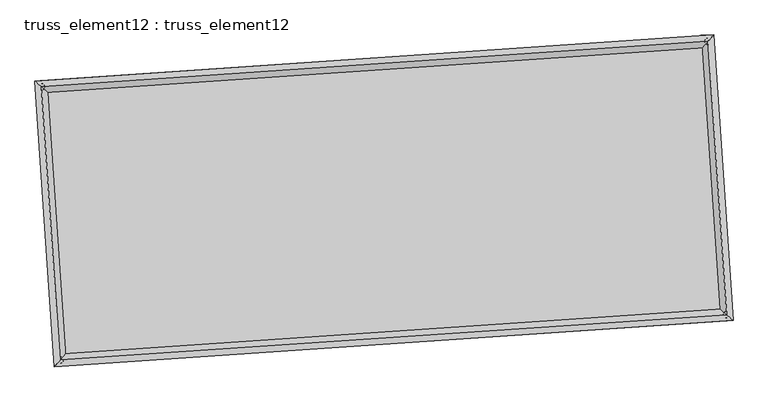
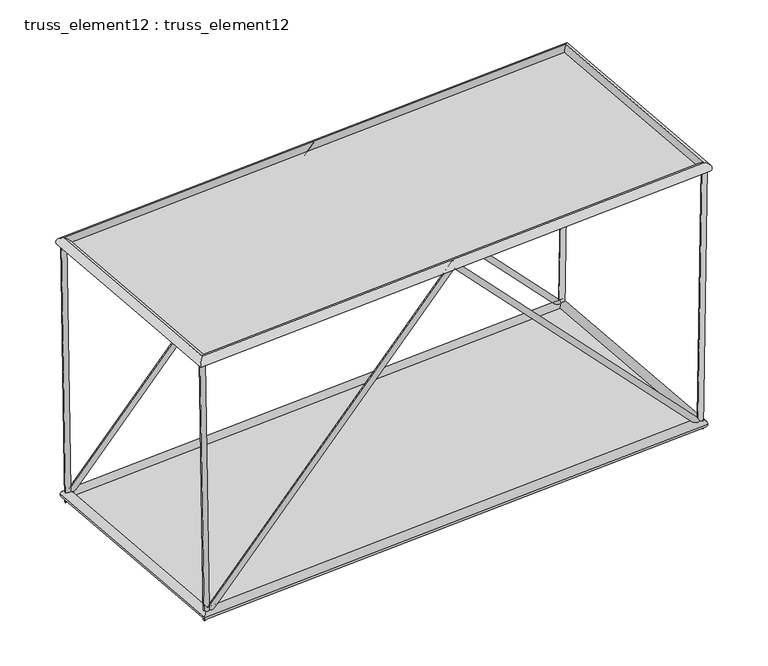
"""IFC4 building model written with IfcOpenShell, lengths in millimetres: plate geometry, truss_element12 : truss_element12."""

import ifcopenshell
import ifcopenshell.guid

model = None  # the IFC model being written
_history = None  # IfcOwnerHistory: only IFC2X3 demands one
_inside = {}  # id of a spatial element -> (the spatial element, [elements in it])
_under = {}  # id of a project, library or spatial element -> (it, [spatial elements below it])
_declared = {}  # id of a project -> (the project, [libraries it declares])
_typed = {}  # id of a type object -> (the type object, [elements of that type])
_made_of = {}  # id of a material, layer set ... -> (it, [elements and type objects made of it])


def new_model(schema):
    """Start an empty IFC model of exactly this schema.

    Asked for "IFC4X3", IfcOpenShell would pick the latest addendum, in which some entities
    have other attributes; the version numbers below select the first issue.
    IFC2X3 requires an IfcOwnerHistory on every rooted entity: one is made here for all.
    """
    global model, _history
    if schema == "IFC4X3":
        model = ifcopenshell.file(schema_version=(4, 3, 0, 0))
    else:
        model = ifcopenshell.file(schema=schema)
    _inside.clear()
    _under.clear()
    _declared.clear()
    _typed.clear()
    _made_of.clear()
    _history = None
    if model.schema == "IFC2X3":
        org = make("IfcOrganization", Name="unknown")
        user = make(
            "IfcPersonAndOrganization",
            ThePerson=make("IfcPerson", FamilyName="unknown"),
            TheOrganization=org,
        )
        app = make(
            "IfcApplication",
            ApplicationDeveloper=org,
            Version="unknown",
            ApplicationFullName="unknown",
            ApplicationIdentifier="unknown",
        )
        _history = make(
            "IfcOwnerHistory",
            OwningUser=user,
            OwningApplication=app,
            ChangeAction="ADDED",
            CreationDate=0,
        )
    return model


def make(cls, **values):
    """One entity of the class cls with the attributes given. An attribute that is None is left unset."""
    return model.create_entity(
        cls, **{name: value for name, value in values.items() if value is not None}
    )


def rooted(cls, **values):
    """An entity with a GlobalId (a new one), such as an element, a storey or a relation."""
    return make(cls, GlobalId=ifcopenshell.guid.new(), OwnerHistory=_history, **values)


def si_unit(unit_type, name, prefix=None):
    """IfcSIUnit, for example si_unit("LENGTHUNIT", "METRE", prefix="MILLI")."""
    return make("IfcSIUnit", UnitType=unit_type, Prefix=prefix, Name=name)


def assignment(units):
    """IfcUnitAssignment: the units of a project."""
    return None if units is None else make("IfcUnitAssignment", Units=units)


def point(xyz):
    """IfcCartesianPoint."""
    return None if xyz is None else make("IfcCartesianPoint", Coordinates=xyz)


def direction(xyz):
    """IfcDirection."""
    return None if xyz is None else make("IfcDirection", DirectionRatios=xyz)


def frame(location, z_axis=None, x_axis=None):
    """IfcAxis2Placement3D, a coordinate frame: its origin and axes. An axis left out is left unset."""
    return make(
        "IfcAxis2Placement3D",
        Location=point(location),
        Axis=direction(z_axis),
        RefDirection=direction(x_axis),
    )


def origin():
    """The frame at (0, 0, 0) with its axes left unset."""
    return frame((0.0, 0.0, 0.0))


def origin_with_axes():
    """The frame at (0, 0, 0) with the z axis (0, 0, 1) and the x axis (1, 0, 0) written out."""
    return frame((0.0, 0.0, 0.0), z_axis=(0.0, 0.0, 1.0), x_axis=(1.0, 0.0, 0.0))


def place(relative_to, where):
    """IfcLocalPlacement: puts the frame where relative to a parent placement (None: the world)."""
    return make(
        "IfcLocalPlacement", PlacementRelTo=relative_to, RelativePlacement=where
    )


def context(
    kind, dimensions, precision=None, world=None, true_north=None, identifier=None
):
    """IfcGeometricRepresentationContext, for example the 3D "Model" context."""
    return make(
        "IfcGeometricRepresentationContext",
        ContextIdentifier=identifier,
        ContextType=kind,
        CoordinateSpaceDimension=dimensions,
        Precision=precision,
        WorldCoordinateSystem=world,
        TrueNorth=true_north,
    )


def project(units=None, contexts=None):
    """IfcProject with its units and contexts."""
    return rooted(
        "IfcProject",
        Name="project",
        RepresentationContexts=contexts,
        UnitsInContext=assignment(units),
    )


def spatial(cls, under=None, at=None, **own):
    """A site, building, storey or space (cls), placed at a placement, below another one or the project."""
    s = rooted(cls, ObjectPlacement=at, **own)
    if under is not None:
        _under.setdefault(under.id(), (under, []))[1].append(s)
    return s


def polyline(points):
    """IfcPolyline through the points."""
    return make("IfcPolyline", Points=[point(p) for p in points])


def circle_curve(where, radius):
    """IfcCircle in the frame where."""
    return make("IfcCircle", Position=where, Radius=radius)


def ellipse_curve(where, semi_axis1, semi_axis2):
    """IfcEllipse in the frame where."""
    return make(
        "IfcEllipse", Position=where, SemiAxis1=semi_axis1, SemiAxis2=semi_axis2
    )


def outline(outer, holes=None, kind="AREA"):
    """IfcArbitraryClosedProfileDef: a profile drawn as a closed curve; with holes, ...WithVoids."""
    if holes is None:
        return make("IfcArbitraryClosedProfileDef", ProfileType=kind, OuterCurve=outer)
    return make(
        "IfcArbitraryProfileDefWithVoids",
        ProfileType=kind,
        OuterCurve=outer,
        InnerCurves=holes,
    )


def extrude(swept, where, along, depth):
    """IfcExtrudedAreaSolid: the profile swept, set in the frame where, extruded along a direction by depth."""
    return make(
        "IfcExtrudedAreaSolid",
        SweptArea=swept,
        Position=where,
        ExtrudedDirection=direction(along),
        Depth=depth,
    )


def shape(context_of_items, identifier, shape_type, items):
    """IfcShapeRepresentation: the items that make up one representation, for example the "Body"."""
    return make(
        "IfcShapeRepresentation",
        ContextOfItems=context_of_items,
        RepresentationIdentifier=identifier,
        RepresentationType=shape_type,
        Items=items,
    )


def source(mapping_origin, context_of_items, identifier, shape_type, items):
    """IfcRepresentationMap: a shape defined once, which mapped items show again and again."""
    return make(
        "IfcRepresentationMap",
        MappingOrigin=mapping_origin,
        MappedRepresentation=shape(context_of_items, identifier, shape_type, items),
    )


def transform(
    local_origin,
    x_axis=None,
    y_axis=None,
    z_axis=None,
    scale=None,
    scale2=None,
    scale3=None,
    uniform=True,
):
    """IfcCartesianTransformationOperator3D, or its non-uniform kind. x_axis, y_axis, z_axis: its Axis1, 2, 3."""
    if uniform:
        return make(
            "IfcCartesianTransformationOperator3D",
            Axis1=direction(x_axis),
            Axis2=direction(y_axis),
            LocalOrigin=point(local_origin),
            Scale=scale,
            Axis3=direction(z_axis),
        )
    return make(
        "IfcCartesianTransformationOperator3DnonUniform",
        Axis1=direction(x_axis),
        Axis2=direction(y_axis),
        LocalOrigin=point(local_origin),
        Scale=scale,
        Axis3=direction(z_axis),
        Scale2=scale2,
        Scale3=scale3,
    )


def mapped(mapping_source, mapping_target):
    """IfcMappedItem: shows the shape of a source again, moved by a transform."""
    return make(
        "IfcMappedItem", MappingSource=mapping_source, MappingTarget=mapping_target
    )


def made_of(thing, what):
    """Note that an element or type object is made of a material, layer set ...; save() writes the relation."""
    if what is not None:
        _made_of.setdefault(what.id(), (what, []))[1].append(thing)
    return thing


def element(
    cls,
    number,
    at=None,
    inside=None,
    cuts=None,
    type_object=None,
    material=None,
    context=None,
    identifier="Body",
    shape_type=None,
    held_by="IfcProductDefinitionShape",
    body=None,
    shapes=None,
    **own,
):
    """One element of the class cls, such as IfcWall. Its Tag is "e" and its number.

    at: its placement. inside: the storey or other place that contains it. cuts: it is an
    opening in that element (IfcRelVoidsElement). A single representation is given by context,
    identifier, shape_type and body (its items); several are given by shapes. held_by: the class
    of the entity that holds the representations. save() writes the other relations.
    """
    e = rooted(cls, Tag="e%d" % number, ObjectPlacement=at, **own)
    if body is not None:
        shapes = [shape(context, identifier, shape_type, body)]
    if shapes is not None:
        e.Representation = make(held_by, Representations=shapes)
    if inside is not None:
        _inside.setdefault(inside.id(), (inside, []))[1].append(e)
    if cuts is not None:
        rooted(
            "IfcRelVoidsElement", RelatingBuildingElement=cuts, RelatedOpeningElement=e
        )
    if type_object is not None:
        _typed.setdefault(type_object.id(), (type_object, []))[1].append(e)
    return made_of(e, material)


def aggregate(whole, parts):
    """IfcRelAggregates: a whole, such as a stair, and the parts it consists of."""
    return rooted("IfcRelAggregates", RelatingObject=whole, RelatedObjects=parts)


def save(model, path):
    """Write the relations noted so far, then the file.

    IfcRelAggregates (storeys below a building ...), IfcRelContainedInSpatialStructure (elements
    in a storey), IfcRelDefinesByType, IfcRelAssociatesMaterial and IfcRelDeclares: one each for
    every whole, place, type object, material and project.
    """
    for whole, parts in _under.values():
        aggregate(whole, parts)
    for where, things in _inside.values():
        rooted(
            "IfcRelContainedInSpatialStructure",
            RelatedElements=things,
            RelatingStructure=where,
        )
    for kind, things in _typed.values():
        rooted("IfcRelDefinesByType", RelatedObjects=things, RelatingType=kind)
    for what, things in _made_of.values():
        rooted("IfcRelAssociatesMaterial", RelatedObjects=things, RelatingMaterial=what)
    for by, libraries in _declared.values():
        rooted("IfcRelDeclares", RelatingContext=by, RelatedDefinitions=libraries)
    model.write(path)


def plane_surface(at):
    """IfcPlane: the flat surface through the origin of the frame at, square to its z axis."""
    return make("IfcPlane", Position=at)


def cylinder_surface(at, radius):
    """IfcCylindricalSurface: all points at the distance radius from the z axis of the frame at."""
    return make("IfcCylindricalSurface", Position=at, Radius=radius)


def advanced_brep(points, edges, surfaces, faces):
    """IfcAdvancedBrep: a solid bounded by faces that lie on surfaces and meet in shared edges.

    An edge is (start, end): straight between two places in points (the first is 0);
    or (start, end, curve); or (start, end, curve, False) where it runs against its curve.
    A face is (place in surfaces, loops), or (place, loops, False) where it looks against
    its surface's normal. A loop lists edges by number (the first is 1), with a minus sign
    where the edge is run from its end to its start. The first loop is the outer one.
    """
    corners = [point(p) for p in points]
    vertices = [make("IfcVertexPoint", VertexGeometry=c) for c in corners]
    made = []
    for start, end, *more in edges:
        made.append(
            make(
                "IfcEdgeCurve",
                EdgeStart=vertices[start],
                EdgeEnd=vertices[end],
                EdgeGeometry=more[0] if more else make("IfcPolyline", Points=[corners[start], corners[end]]),
                SameSense=more[1] if len(more) > 1 else True,
            )
        )
    hull = []
    for where, loops, *sense in faces:
        bounds = []
        for j, loop in enumerate(loops):
            ring = [make("IfcOrientedEdge", EdgeElement=made[abs(k) - 1], Orientation=k > 0) for k in loop]
            bounds.append(
                make(
                    "IfcFaceOuterBound" if j == 0 else "IfcFaceBound",
                    Bound=make("IfcEdgeLoop", EdgeList=ring),
                    Orientation=True,
                )
            )
        hull.append(make("IfcAdvancedFace", Bounds=bounds, FaceSurface=surfaces[where], SameSense=sense[0] if sense else True))
    return make("IfcAdvancedBrep", Outer=make("IfcClosedShell", CfsFaces=hull))


def truss_element12_truss_element12_1bbcfac7(model_context):
    return source(origin(), model_context, "Body", "SolidModel", [
        advanced_brep(
        [(-3746.2779315, 2270.677949, 5000.1488437), (-3845.3680681, 2257.3176242, 4998.522018), (-3666.9216571, 2276.0889517, 122.1113591), (-3762.0652257, 2262.9977284, -122.1113591), (1064.4228838, 2598.7013505, 5071.4427935), (1064.8605805, 2592.1274502, 4927.2050495), (5794.3942317, 2921.2201164, 122.1016693), (5890.3667453, 2921.1603721, -122.1016693), (5875.1134246, 2926.7240513, 5000.1397912), (5975.0995037, 2926.9379768, 4998.4850331)],
        [
            (0, 1, circle_curve(frame((-3795.8229998, 2263.9977866, 4999.3354308), z_axis=(-0.016265911675968303, -0.0011091106846651264, 0.9998670861623754), x_axis=(-0.1336035338535352, 0.9910342788842121, -0.0010741593443196402)), 50.0)),
            (1, 0, circle_curve(frame((-3795.8229998, 2263.9977866, 4999.3354308), z_axis=(-0.016265911675968303, -0.0011091106846651264, 0.9998670861623754), x_axis=(-0.1336035338535352, 0.9910342788842121, -0.0010741593443196402)), 50.0)),
            (0, 2),
            (2, 3, ellipse_curve(frame((-3714.4934414, 2269.54334, 0.0), z_axis=(-0.9287646394568875, -0.06332893019963927, 0.36522005845009003), x_axis=(0.36437398822915085, 0.02484527714214224, 0.9309212151979955)), 131.4582279, 50.0)),
            (3, 1),
            (3, 2, ellipse_curve(frame((-3714.4934414, 2269.54334, 0.0), z_axis=(-0.9287646394568875, -0.06332893019963927, 0.36522005845009003), x_axis=(0.36437398822915085, 0.02484527714214224, 0.9309212151979955)), 131.4582279, 50.0)),
            (2, 4),
            (4, 5, ellipse_curve(frame((1064.6417322, 2595.4144003, 4999.3239215), z_axis=(-0.9976833934171915, -0.06802823804748175, 7.299118212849759e-05), x_axis=(-7.282209046969254e-05, -4.9654615264680074e-06, -0.9999999973361436)), 72.2759091, 50.0)),
            (5, 3),
            (5, 4, ellipse_curve(frame((1064.6417322, 2595.4144003, 4999.3239215), z_axis=(-0.9976833934171915, -0.06802823804748175, 7.299118212849759e-05), x_axis=(-7.282209046969254e-05, -4.9654615264680074e-06, -0.9999999973361436)), 72.2759091, 50.0)),
            (4, 6),
            (6, 7, ellipse_curve(frame((5842.3804885, 2921.1902443, 0.0), z_axis=(-0.9288422213363277, -0.06333422021308223, -0.3650217862169288), x_axis=(-0.3641761753142233, -0.02483178903143046, 0.930998977221244)), 131.4368172, 50.0)),
            (7, 5),
            (7, 6, ellipse_curve(frame((5842.3804885, 2921.1902443, 0.0), z_axis=(-0.9288422213363277, -0.06333422021308223, -0.3650217862169288), x_axis=(-0.3641761753142233, -0.02483178903143046, 0.930998977221244)), 131.4368172, 50.0)),
            (8, 9, circle_curve(frame((5925.1064641, 2926.8310141, 4999.3124122), z_axis=(0.016545195126702994, 0.0011281539615151874, 0.9998624824378893), x_axis=(-0.0021576295961431924, 0.9999970754228623, -0.0010926025114963022)), 50.0)),
            (9, 8, circle_curve(frame((5925.1064641, 2926.8310141, 4999.3124122), z_axis=(0.016545195126702994, 0.0011281539615151874, 0.9998624824378893), x_axis=(-0.0021576295961431924, 0.9999970754228623, -0.0010926025114963022)), 50.0)),
            (6, 8),
            (9, 7),
        ],
        [
            plane_surface(frame((-3795.8229998, 2313.9977559, 4999.3908937), z_axis=(-0.016265911675968123, -0.0011091106846617949, 0.9998670861623753), x_axis=(0.9998677013072027, -1.8043083511720685e-05, 0.01626590166875275))),
            cylinder_surface(frame((-3795.8229998, 2263.9977866, 4999.3354308), z_axis=(-0.016265911675968303, -0.0011091106846651264, 0.9998670861623754), x_axis=(-0.1336035338535352, 0.9910342788842121, -0.0010741593443196402)), 50.0),
            cylinder_surface(frame((-3714.4934414, 2269.54334, 0.0), z_axis=(-0.6902434140818179, -0.04706507454537663, -0.7220449487910807), x_axis=(-0.020419087296308105, 0.9987518960405878, -0.045581915595078945)), 50.0),
            cylinder_surface(frame((1064.6417322, 2595.4144003, 4999.3239215), z_axis=(-0.6901382450820931, -0.04705790347107014, 0.7221459384334419), x_axis=(-0.11534841177711228, 0.9922790262643878, -0.045574970502419106)), 50.0),
            plane_surface(frame((5925.1064641, 2876.8310459, 4999.3688276), z_axis=(0.01654519512670156, 0.0011281539615101215, 0.9998624824378892), x_axis=(0.9998631188908906, -1.8668082734762968e-05, -0.016545184595020874))),
            cylinder_surface(frame((5842.3804885, 2921.1902443, 0.0), z_axis=(-0.016545195126702994, -0.0011281539615151874, -0.9998624824378893), x_axis=(-0.0021576295961431924, 0.9999970754228623, -0.0010926025114963022)), 50.0),
        ],
        [
            (0, [[1, 2]]),
            (1, [[-1, 3, 4, 5]]),
            (1, [[-2, -5, 6, -3]]),
            (2, [[-4, 7, 8, 9]]),
            (2, [[-6, -9, 10, -7]]),
            (3, [[-8, 11, 12, 13]]),
            (3, [[-10, -13, 14, -11]]),
            (4, [[15, 16]]),
            (5, [[-12, 17, -16, 18]]),
            (5, [[-14, -18, -15, -17]]),
        ],
    ),
        advanced_brep(
        [(-3474.1649786, -1720.0556353, 5000.1488437), (-3573.2551151, -1733.4159601, 4998.522018), (-3394.8087042, -1714.6446326, 122.1113591), (-3489.9522728, -1727.7358559, -122.1113591), (1336.5358367, -1392.0322338, 5071.4427935), (1336.9735335, -1398.6061341, 4927.2050495), (6066.5071846, -1069.5134679, 122.1016693), (6162.4796982, -1069.5732122, -122.1016693), (6147.2263775, -1064.009533, 5000.1397912), (6247.2124566, -1063.7956075, 4998.4850331)],
        [
            (0, 1, circle_curve(frame((-3523.7100469, -1726.7357977, 4999.3354308), z_axis=(-0.01626591167596829, -0.0011091106846651422, 0.9998670861623754), x_axis=(-0.13360353385353582, 0.991034278884212, -0.0010741593443196332)), 50.0)),
            (1, 0, circle_curve(frame((-3523.7100469, -1726.7357977, 4999.3354308), z_axis=(-0.01626591167596829, -0.0011091106846651422, 0.9998670861623754), x_axis=(-0.13360353385353582, 0.991034278884212, -0.0010741593443196332)), 50.0)),
            (0, 2),
            (2, 3, ellipse_curve(frame((-3442.3804885, -1721.1902443, 0.0), z_axis=(-0.9287646394568875, -0.06332893019963957, 0.36522005845009003), x_axis=(0.36437398822915085, 0.02484527714214235, 0.9309212151979955)), 131.4582279, 50.0)),
            (3, 1),
            (3, 2, ellipse_curve(frame((-3442.3804885, -1721.1902443, 0.0), z_axis=(-0.9287646394568875, -0.06332893019963957, 0.36522005845009003), x_axis=(0.36437398822915085, 0.02484527714214235, 0.9309212151979955)), 131.4582279, 50.0)),
            (2, 4),
            (4, 5, ellipse_curve(frame((1336.7546851, -1395.319184, 4999.3239215), z_axis=(-0.9976833934171915, -0.06802823804748206, 7.299118212825683e-05), x_axis=(-7.282209046923131e-05, -4.965461526419962e-06, -0.9999999973361436)), 72.2759091, 50.0)),
            (5, 3),
            (5, 4, ellipse_curve(frame((1336.7546851, -1395.319184, 4999.3239215), z_axis=(-0.9976833934171915, -0.06802823804748206, 7.299118212825683e-05), x_axis=(-7.282209046923131e-05, -4.965461526419962e-06, -0.9999999973361436)), 72.2759091, 50.0)),
            (4, 6),
            (6, 7, ellipse_curve(frame((6114.4934414, -1069.54334, 0.0), z_axis=(-0.9288422213363275, -0.06333422021308248, -0.3650217862169293), x_axis=(-0.3641761753142236, -0.024831789031430622, 0.930998977221244)), 131.4368172, 50.0)),
            (7, 5),
            (7, 6, ellipse_curve(frame((6114.4934414, -1069.54334, 0.0), z_axis=(-0.9288422213363275, -0.06333422021308248, -0.3650217862169293), x_axis=(-0.3641761753142236, -0.024831789031430622, 0.930998977221244)), 131.4368172, 50.0)),
            (8, 9, circle_curve(frame((6197.2194171, -1063.9025702, 4999.3124122), z_axis=(0.016545195126702262, 0.0011281539615151067, 0.9998624824378893), x_axis=(-0.0021576295961430463, 0.9999970754228623, -0.0010926025114962256)), 50.0)),
            (9, 8, circle_curve(frame((6197.2194171, -1063.9025702, 4999.3124122), z_axis=(0.016545195126702262, 0.0011281539615151067, 0.9998624824378893), x_axis=(-0.0021576295961430463, 0.9999970754228623, -0.0010926025114962256)), 50.0)),
            (6, 8),
            (9, 7),
        ],
        [
            plane_surface(frame((-3523.7100469, -1676.7358284, 4999.3908937), z_axis=(-0.016265911675968123, -0.001109110684661801, 0.9998670861623753), x_axis=(0.9998677013072027, -1.8043083511720685e-05, 0.01626590166875275))),
            cylinder_surface(frame((-3523.7100469, -1726.7357977, 4999.3354308), z_axis=(-0.01626591167596829, -0.0011091106846651422, 0.9998670861623754), x_axis=(-0.13360353385353582, 0.991034278884212, -0.0010741593443196332)), 50.0),
            cylinder_surface(frame((-3442.3804885, -1721.1902443, 0.0), z_axis=(-0.690243414081818, -0.04706507454537685, -0.7220449487910808), x_axis=(-0.020419087296308168, 0.9987518960405878, -0.045581915595079174)), 50.0),
            cylinder_surface(frame((1336.7546851, -1395.319184, 4999.3239215), z_axis=(-0.6901382450820935, -0.0470579034710704, 0.7221459384334415), x_axis=(-0.1153484117771128, 0.9922790262643877, -0.04557497050241935)), 50.0),
            plane_surface(frame((6197.2194171, -1113.9025384, 4999.3688276), z_axis=(0.016545195126701558, 0.001128153961510126, 0.9998624824378892), x_axis=(0.9998631188908906, -1.866808273431888e-05, -0.016545184595020874))),
            cylinder_surface(frame((6114.4934414, -1069.54334, 0.0), z_axis=(-0.016545195126702262, -0.0011281539615151067, -0.9998624824378893), x_axis=(-0.0021576295961430463, 0.9999970754228623, -0.0010926025114962256)), 50.0),
        ],
        [
            (0, [[1, 2]]),
            (1, [[-1, 3, 4, 5]]),
            (1, [[-2, -5, 6, -3]]),
            (2, [[-4, 7, 8, 9]]),
            (2, [[-6, -9, 10, -7]]),
            (3, [[-8, 11, 12, 13]]),
            (3, [[-10, -13, 14, -11]]),
            (4, [[15, 16]]),
            (5, [[-12, 17, -16, 18]]),
            (5, [[-14, -18, -15, -17]]),
        ],
    ),
        advanced_brep(
        [(-3523.7160635, -1726.7424662, 4909.335431), (-3523.7040302, -1726.7291292, 5089.3354306), (-3795.8161337, 2263.9919966, 5089.3354306), (-3795.8298659, 2264.0035767, 4909.335431), (5925.1008717, 2926.8243745, 5089.312412), (5925.1120565, 2926.8376536, 4909.3124124), (6197.2129752, -1063.8967513, 5089.312412), (6197.2258589, -1063.9083892, 4909.3124124)],
        [
            (0, 1, ellipse_curve(frame((-3523.7100469, -1726.7357977, 4999.3354308), z_axis=(-0.7535719234034886, 0.6573654662782159, 1.670510786331496e-06), x_axis=(-0.657365466276113, -0.7535719234053231, 1.6705107863314674e-06)), 127.2792206, 90.0)),
            (1, 2),
            (2, 3, ellipse_curve(frame((-3795.8229998, 2263.9977866, 4999.3354308), z_axis=(-0.657365466276113, -0.7535719234053231, 1.6705107863314422e-06), x_axis=(0.7535719234034887, -0.6573654662782157, -1.6705107863314712e-06)), 127.2792206, 90.0)),
            (3, 0),
            (1, 0, ellipse_curve(frame((-3523.7100469, -1726.7357977, 4999.3354308), z_axis=(-0.7535719234034886, 0.6573654662782159, 1.670510786331496e-06), x_axis=(-0.657365466276113, -0.7535719234053231, 1.6705107863314674e-06)), 127.2792206, 90.0)),
            (3, 2, ellipse_curve(frame((-3795.8229998, 2263.9977866, 4999.3354308), z_axis=(-0.657365466276113, -0.7535719234053231, 1.6705107863314422e-06), x_axis=(0.7535719234034887, -0.6573654662782157, -1.6705107863314712e-06)), 127.2792206, 90.0)),
            (2, 4),
            (4, 5, ellipse_curve(frame((5925.1064641, 2926.8310141, 4999.3124122), z_axis=(-0.7535719234034886, 0.6573654662782158, 1.670510786331446e-06), x_axis=(-0.657365466276113, -0.7535719234053229, 1.6705107863314674e-06)), 127.2792206, 90.0)),
            (5, 3),
            (5, 4, ellipse_curve(frame((5925.1064641, 2926.8310141, 4999.3124122), z_axis=(-0.7535719234034886, 0.6573654662782158, 1.670510786331446e-06), x_axis=(-0.657365466276113, -0.7535719234053229, 1.6705107863314674e-06)), 127.2792206, 90.0)),
            (4, 6),
            (6, 7, ellipse_curve(frame((6197.2194171, -1063.9025702, 4999.3124122), z_axis=(0.6573654662761127, 0.7535719234053232, -1.6705107863314917e-06), x_axis=(-0.7535719234034888, 0.6573654662782156, 1.6705107863314714e-06)), 127.2792206, 90.0)),
            (7, 5),
            (7, 6, ellipse_curve(frame((6197.2194171, -1063.9025702, 4999.3124122), z_axis=(0.6573654662761127, 0.7535719234053232, -1.6705107863314917e-06), x_axis=(-0.7535719234034888, 0.6573654662782156, 1.6705107863314714e-06)), 127.2792206, 90.0)),
            (6, 1),
            (0, 7),
        ],
        [
            cylinder_surface(frame((-3523.7100469, -1726.7357977, 4999.3354308), z_axis=(0.06802823822869979, -0.9976833960748768, 0.0), x_axis=(-0.9976833935077207, -0.06802823805365518, 7.173725476019441e-05)), 90.0),
            cylinder_surface(frame((-3795.8229998, 2263.9977866, 4999.3354308), z_axis=(-0.9976833960720926, -0.06802823822851069, 2.3624590101204896e-06), x_axis=(-0.06802823790147983, 0.9976833936851698, 6.937479575575899e-05)), 90.0),
            cylinder_surface(frame((5925.1064641, 2926.8310141, 4999.3124122), z_axis=(-0.06802823822870002, 0.9976833960748767, 0.0), x_axis=(0.9976833938347516, 0.0680282380759544, 6.701233675132358e-05)), 90.0),
            cylinder_surface(frame((6197.2194171, -1063.9025702, 4999.3124122), z_axis=(0.9976833960720927, 0.0680282382285108, -2.362459010120525e-06), x_axis=(0.0680282382285108, -0.9976833936628708, 6.937479575575899e-05)), 90.0),
        ],
        [
            (0, [[1, 2, 3, 4]]),
            (0, [[5, -4, 6, -2]]),
            (1, [[-3, 7, 8, 9]]),
            (1, [[-6, -9, 10, -7]]),
            (2, [[-8, 11, 12, 13]]),
            (2, [[-10, -13, 14, -11]]),
            (3, [[-12, 15, -1, 16]]),
            (3, [[-14, -16, -5, -15]]),
        ],
    ),
        advanced_brep(
        [(-3358.7115243, -1625.2761972, 0.0), (-3526.0494527, -1817.1042913, 0.0), (-3810.4074885, 2353.2123043, 0.0), (-3618.5793943, 2185.8743758, 0.0), (5926.0494527, 3017.1042913, 0.0), (5758.7115243, 2825.2761972, 0.0), (6210.4074885, -1153.2123043, 0.0), (6018.5793943, -985.8743758, 0.0)],
        [
            (0, 1, ellipse_curve(frame((-3442.3804885, -1721.1902443, 0.0), z_axis=(-0.7535719234054563, 0.6573654662780828, 0.0), x_axis=(-0.6573654662780828, -0.7535719234054562, 0.0)), 127.2792206, 90.0)),
            (1, 2),
            (2, 3, ellipse_curve(frame((-3714.4934414, 2269.54334, 0.0), z_axis=(-0.6573654662780828, -0.7535719234054563, 0.0), x_axis=(0.7535719234054564, -0.6573654662780826, 0.0)), 127.2792206, 90.0)),
            (3, 0),
            (1, 0, ellipse_curve(frame((-3442.3804885, -1721.1902443, 0.0), z_axis=(-0.7535719234054563, 0.6573654662780828, 0.0), x_axis=(-0.6573654662780828, -0.7535719234054562, 0.0)), 127.2792206, 90.0)),
            (3, 2, ellipse_curve(frame((-3714.4934414, 2269.54334, 0.0), z_axis=(-0.6573654662780828, -0.7535719234054563, 0.0), x_axis=(0.7535719234054564, -0.6573654662780826, 0.0)), 127.2792206, 90.0)),
            (2, 4),
            (4, 5, ellipse_curve(frame((5842.3804885, 2921.1902443, 0.0), z_axis=(-0.7535719234054562, 0.6573654662780827, 0.0), x_axis=(-0.6573654662780829, -0.7535719234054562, 0.0)), 127.2792206, 90.0)),
            (5, 3),
            (5, 4, ellipse_curve(frame((5842.3804885, 2921.1902443, 0.0), z_axis=(-0.7535719234054562, 0.6573654662780827, 0.0), x_axis=(-0.6573654662780829, -0.7535719234054562, 0.0)), 127.2792206, 90.0)),
            (4, 6),
            (6, 7, ellipse_curve(frame((6114.4934414, -1069.54334, 0.0), z_axis=(0.6573654662780828, 0.7535719234054563, 0.0), x_axis=(-0.7535719234054563, 0.6573654662780827, 0.0)), 127.2792206, 90.0)),
            (7, 5),
            (7, 6, ellipse_curve(frame((6114.4934414, -1069.54334, 0.0), z_axis=(0.6573654662780828, 0.7535719234054563, 0.0), x_axis=(-0.7535719234054563, 0.6573654662780827, 0.0)), 127.2792206, 90.0)),
            (6, 1),
            (0, 7),
        ],
        [
            cylinder_surface(frame((-3442.3804885, -1721.1902443, 0.0), z_axis=(0.0680282382286984, -0.9976833960748769, 0.0), x_axis=(-0.9976833960748769, -0.0680282382286984, 0.0)), 90.0),
            cylinder_surface(frame((-3714.4934414, 2269.54334, 0.0), z_axis=(-0.9976833960748769, -0.06802823822869901, 0.0), x_axis=(-0.06802823822869901, 0.9976833960748769, 0.0)), 90.0),
            cylinder_surface(frame((5842.3804885, 2921.1902443, 0.0), z_axis=(-0.06802823822869834, 0.9976833960748769, 0.0), x_axis=(0.9976833960748769, 0.06802823822869834, 0.0)), 90.0),
            cylinder_surface(frame((6114.4934414, -1069.54334, 0.0), z_axis=(0.9976833960748768, 0.0680282382286991, 0.0), x_axis=(0.0680282382286991, -0.9976833960748768, 0.0)), 90.0),
        ],
        [
            (0, [[1, 2, 3, 4]]),
            (0, [[5, -4, 6, -2]]),
            (1, [[-3, 7, 8, 9]]),
            (1, [[-6, -9, 10, -7]]),
            (2, [[-8, 11, 12, 13]]),
            (2, [[-10, -13, 14, -11]]),
            (3, [[-12, 15, -1, 16]]),
            (3, [[-14, -16, -5, -15]]),
        ],
    ),
        extrude(outline(polyline([(-3442.3804885, -1721.1902443), (-3714.4934414, 2269.54334), (5842.3804885, 2921.1902443), (6114.4934414, -1069.54334), (-3442.3804885, -1721.1902443)])), origin_with_axes(), (0.0, 0.0, 1.0), 20.0),
        extrude(outline(polyline([(-2000.0, 4871.7506486), (2000.0, 4871.7506486), (2000.0, -4871.7506486), (-2000.0, -4871.7506487), (-2000.0, 4871.7506486)])), frame((1200.6982086, 600.0476082, 4999.3239215), z_axis=(2.3569861283047194e-06, 1.6071392434601366e-07, 0.9999999999972095), x_axis=(-0.06802823822869873, 0.9976833960748768, 0.0)), (0.0, 0.0, 1.0), 20.0),
    ])


if __name__ == "__main__":
    model = new_model("IFC4")
    model_context = context("Model", 3, world=origin())
    ifc_project = project(units=[si_unit("LENGTHUNIT", "METRE", prefix="MILLI")], contexts=[model_context])
    site = spatial("IfcSite", under=ifc_project)
    building = spatial("IfcBuilding", under=site)
    placement = place(None, origin())
    truss_element12_truss_element12_shape = truss_element12_truss_element12_1bbcfac7(model_context)
    element("IfcPlate", 1, ObjectType="truss_element12 : truss_element12", at=placement, inside=building, context=model_context, shape_type="MappedRepresentation", body=[
        mapped(truss_element12_truss_element12_shape, transform((0.0, 0.0, 0.0), x_axis=(1.0, 0.0, 0.0), y_axis=(0.0, 1.0, 0.0), z_axis=(0.0, 0.0, 1.0))),
    ])
    save(model, "model.ifc")

# Revit data of these elements
# Type "truss_element12 : truss_element12"
#   steellbar1 = 90 mm
#   steelbar2 = 50 mm
#   offset1 = 5000 mm
#   M = Default Roof
# Element 1 (IfcPlate, "truss_element12 : truss_element12")
#   Materials on its faces: "Default Roof"
# Materials
#   "Default Roof": class "Miscellaneous", colour RGB 0 127 0, transparency 0, Comments = "Rendering appearance not upgraded Rendering appearance not upgraded ", Cost = 0
